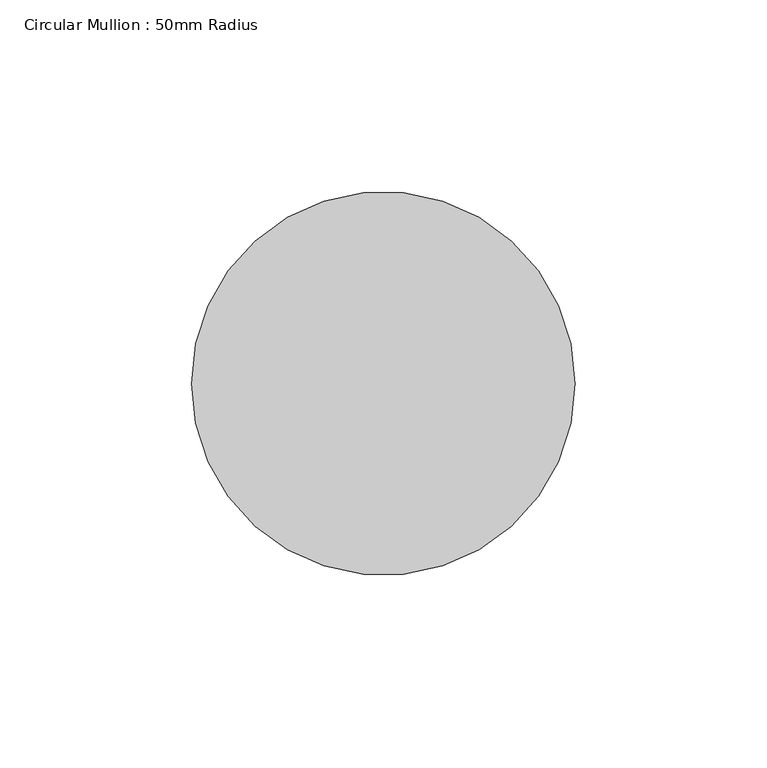
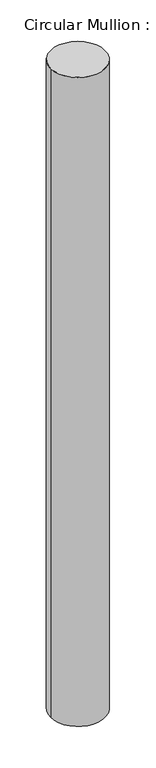
"""IFC4 building model written with IfcOpenShell, lengths in millimetres: member geometry, Circular Mullion : 50mm Radius."""

from ifc_helpers import new_model, si_unit, point, frame, origin, origin_2d, place, context, project, spatial, circle_curve, trimmed, segment, composite_curve, outline, extrude, source, transform, mapped, element, save


def circular_mullion_50mm_radius_46256dbf(model_context):
    return source(origin(), model_context, "Body", "SweptSolid", [
        extrude(outline(composite_curve([segment(trimmed(circle_curve(origin_2d(), 50.0), [point((50.0, 0.0))], [point((-50.0, 0.0))], False, "CARTESIAN"), True, "CONTINUOUS"), segment(trimmed(circle_curve(origin_2d(), 50.0), [point((-50.0, 0.0))], [point((50.0, 0.0))], False, "CARTESIAN"), True, "CONTINUOUS")], self_intersect=False)), frame((0.0, 0.0, -1261.9169754), z_axis=(0.0, 0.0, 1.0), x_axis=(1.0, 0.0, 0.0)), (0.0, 0.0, 1.0), 1261.9169754),
    ])


if __name__ == "__main__":
    model = new_model("IFC4")
    model_context = context("Model", 3, world=origin())
    ifc_project = project(units=[si_unit("LENGTHUNIT", "METRE", prefix="MILLI")], contexts=[model_context])
    site = spatial("IfcSite", under=ifc_project)
    building = spatial("IfcBuilding", under=site)
    placement = place(None, origin())
    circular_mullion_50mm_radius_shape = circular_mullion_50mm_radius_46256dbf(model_context)
    element("IfcMember", 1, ObjectType="Circular Mullion : 50mm Radius", at=placement, inside=building, context=model_context, shape_type="MappedRepresentation", body=[
        mapped(circular_mullion_50mm_radius_shape, transform((0.0, 0.0, 0.0), x_axis=(1.0, 0.0, 0.0), y_axis=(0.0, 1.0, 0.0), z_axis=(0.0, 0.0, 1.0))),
    ])
    save(model, "model.ifc")

# Revit data of these elements
# Type "Circular Mullion : 50mm Radius"
#   built-in parameter 1007350 = 0.164042 (stored number, unit not read)
# Element 1 (IfcMember, "Circular Mullion : 50mm Radius")
#   Materials on its faces: "Aluminium"
# Materials
#   "Aluminium": class "Metal", colour RGB 247 247 247, transparency 0, Description = "Aluminium 6061", Cost = 0
